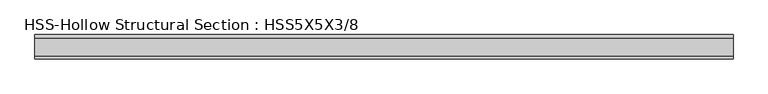
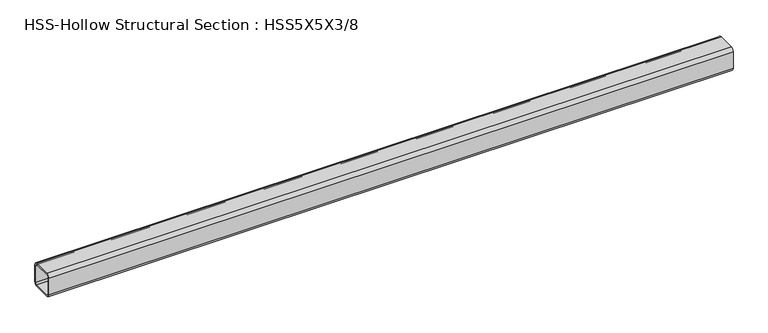
"""IFC4 building model written with IfcOpenShell, lengths in millimetres: member geometry, HSS-Hollow Structural Section : HSS5X5X3/8."""

from ifc_helpers import new_model, si_unit, point, frame, frame_2d, origin, place, context, project, spatial, polyline, circle_curve, trimmed, segment, composite_curve, outline, extrude, source, transform, mapped, element, save


def hss_hollow_structural_section_hss5x5x3_8_dc481f45(model_context):
    return source(origin(), model_context, "Body", "SweptSolid", [
        extrude(outline(composite_curve([segment(polyline([(63.5, 45.7708), (63.5, -45.7708)]), True, "CONTINUOUS"), segment(trimmed(circle_curve(frame_2d((45.7708, -45.7708)), 17.7292), [point((63.5, -45.7708))], [point((45.7708, -63.5))], False, "CARTESIAN"), True, "CONTINUOUS"), segment(polyline([(45.7708, -63.5), (-45.7708, -63.5)]), True, "CONTINUOUS"), segment(trimmed(circle_curve(frame_2d((-45.7708, -45.7708)), 17.7292), [point((-45.7708, -63.5))], [point((-63.5, -45.7708))], False, "CARTESIAN"), True, "CONTINUOUS"), segment(polyline([(-63.5, -45.7708), (-63.5, 45.7708)]), True, "CONTINUOUS"), segment(trimmed(circle_curve(frame_2d((-45.7708, 45.7708)), 17.7292), [point((-63.5, 45.7708))], [point((-45.7708, 63.5))], False, "CARTESIAN"), True, "CONTINUOUS"), segment(polyline([(-45.7708, 63.5), (45.7708, 63.5)]), True, "CONTINUOUS"), segment(trimmed(circle_curve(frame_2d((45.7708, 45.7708)), 17.7292), [point((45.7708, 63.5))], [point((63.5, 45.7708))], False, "CARTESIAN"), True, "CONTINUOUS")], self_intersect=False), holes=[composite_curve([segment(trimmed(circle_curve(frame_2d((-45.7708, 45.7708)), 8.8646), [point((-45.7708, 54.6354))], [point((-54.6354, 45.7708))], True, "CARTESIAN"), True, "CONTINUOUS"), segment(polyline([(-54.6354, 45.7708), (-54.6354, -45.7708)]), True, "CONTINUOUS"), segment(trimmed(circle_curve(frame_2d((-45.7708, -45.7708)), 8.8646), [point((-54.6354, -45.7708))], [point((-45.7708, -54.6354))], True, "CARTESIAN"), True, "CONTINUOUS"), segment(polyline([(-45.7708, -54.6354), (45.7708, -54.6354)]), True, "CONTINUOUS"), segment(trimmed(circle_curve(frame_2d((45.7708, -45.7708)), 8.8646), [point((45.7708, -54.6354))], [point((54.6354, -45.7708))], True, "CARTESIAN"), True, "CONTINUOUS"), segment(polyline([(54.6354, -45.7708), (54.6354, 45.7708)]), True, "CONTINUOUS"), segment(trimmed(circle_curve(frame_2d((45.7708, 45.7708)), 8.8646), [point((54.6354, 45.7708))], [point((45.7708, 54.6354))], True, "CARTESIAN"), True, "CONTINUOUS"), segment(polyline([(45.7708, 54.6354), (-45.7708, 54.6354)]), True, "CONTINUOUS")], self_intersect=False)]), frame((-1806.6414008, 0.0, 0.0), z_axis=(1.0, 0.0, 0.0), x_axis=(0.0, 1.0, 0.0)), (0.0, 0.0, 1.0), 3613.2828016),
    ])


if __name__ == "__main__":
    model = new_model("IFC4")
    model_context = context("Model", 3, world=origin())
    ifc_project = project(units=[si_unit("LENGTHUNIT", "METRE", prefix="MILLI")], contexts=[model_context])
    site = spatial("IfcSite", under=ifc_project)
    building = spatial("IfcBuilding", under=site)
    placement = place(None, origin())
    hss_hollow_structural_section_hss5x5x3_8_shape = hss_hollow_structural_section_hss5x5x3_8_dc481f45(model_context)
    element("IfcMember", 1, ObjectType="HSS-Hollow Structural Section : HSS5X5X3/8", at=placement, inside=building, context=model_context, shape_type="MappedRepresentation", body=[
        mapped(hss_hollow_structural_section_hss5x5x3_8_shape, transform((0.0, 0.0, 0.0), x_axis=(1.0, 0.0, 0.0), y_axis=(0.0, 1.0, 0.0), z_axis=(0.0, 0.0, 1.0))),
    ])
    save(model, "model.ifc")

# Revit data of these elements
# Type "HSS-Hollow Structural Section : HSS5X5X3/8"
#   Assembly Code = "B10"
#   Shape = "Square"
#   W = 22.3
#   Ht = 0' - 5"
#   Length [instance default] = 5' - 0"
#   b = 0' - 5"
#   kr = 0' - 0.698"
#   t = 0' - 0.349"
#   A = 0.0429167 SF
#   Structural Material [instance default] = Steel ASTM A500, Grade B, Rectangular and Square
# Element 1 (IfcMember, "HSS-Hollow Structural Section : HSS5X5X3/8")
#   Materials on its faces: "Steel ASTM A500, Grade B, Rectangular and Square"
# Materials
#   "Steel ASTM A500, Grade B, Rectangular and Square": class "Metal", colour RGB 199 199 199, transparency 0, Description = "Carbon steel", Cost = 0
